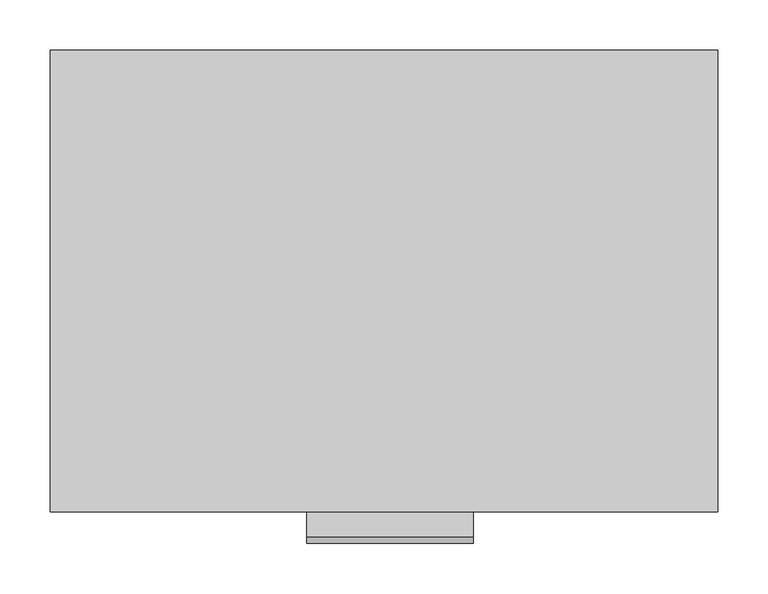
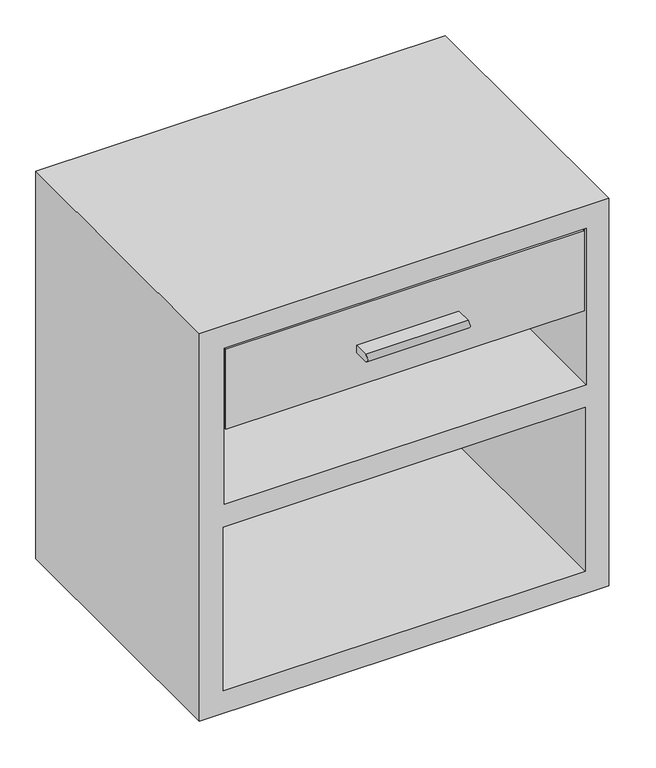
"""IFC4 building model written with IfcOpenShell, lengths in millimetres: furniture geometry, Livia_1_Drawer_Nightstand_20913 : Livia_1_Drawer_Nightstand_20913."""

from ifc_helpers import new_model, si_unit, frame, origin, place, context, project, spatial, faceted_brep, source, transform, mapped, element, save
from ifc_brep_helpers import plane_surface, extruded_surface, spline_curve, advanced_brep


def furniture_23f017af(model_context):
    return source(origin(), model_context, "Body", "SolidModel", [
        advanced_brep(
        [(-76.575761, -228.6, 552.45), (-76.575761, -228.6, 539.75), (-76.575761, -254.0, 539.75), (-76.575761, -254.0, 552.45), (88.524239, -228.6, 552.45), (88.524239, -254.0, 552.45), (88.524239, -254.0, 539.75), (88.524239, -228.6, 539.75)],
        [
            (0, 1),
            (1, 2),
            (2, 3, spline_curve(3, [(-76.575761, -254.0, 539.75), (-76.575761, -261.758833332, 543.737102154), (-76.575761, -261.758833332, 547.970435488), (-76.575761, -254.0, 552.45)], [4, 4], [0.0, 0.04350998662349671])),
            (3, 0),
            (4, 5),
            (5, 6, spline_curve(3, [(88.524239, -254.0, 552.45), (88.524239, -261.758833332, 547.970435488), (88.524239, -261.758833332, 543.737102154), (88.524239, -254.0, 539.75)], [4, 4], [0.0, 0.04350998662349671])),
            (6, 7),
            (7, 4),
            (0, 4),
            (7, 1),
            (6, 2),
            (5, 3),
        ],
        [
            plane_surface(frame((-76.575761, -228.6, 545.7306532), z_axis=(-1.0, 0.0, 0.0), x_axis=(0.0, -1.0, 0.0))),
            plane_surface(frame((88.524239, -228.6, 545.7306532), z_axis=(1.0, 0.0, 0.0), x_axis=(0.0, -1.0, 0.0))),
            plane_surface(frame((-76.575761, -228.6, 552.45), z_axis=(0.0, 1.0, 0.0), x_axis=(1.0, 0.0, 0.0))),
            plane_surface(frame((-76.575761, -228.6, 539.75), z_axis=(0.0, 0.0, -1.0), x_axis=(1.0, 0.0, 0.0))),
            extruded_surface(spline_curve(3, [(88.524239, -254.0, 539.75), (88.524239, -261.758833332, 543.737102154), (88.524239, -261.758833332, 547.970435488), (88.524239, -254.0, 552.45)], [4, 4], [0.0, 0.04350998662349671]), (-165.1, 0.0, 0.0), 165.1),
            plane_surface(frame((-76.575761, -254.0, 552.45), z_axis=(0.0, 0.0, 1.0), x_axis=(1.0, 0.0, 0.0))),
        ],
        [
            (0, [[1, 2, 3, 4]]),
            (1, [[5, 6, 7, 8]]),
            (2, [[-1, 9, -8, 10]]),
            (3, [[-2, -10, -7, 11]]),
            (4, [[-3, -11, -6, 12]]),
            (5, [[-4, -12, -5, -9]]),
        ],
    ),
        faceted_brep([(330.2, -228.6, 0.0), (330.2, -228.6, 660.4), (-330.2, -228.6, 660.4), (-330.2, -228.6, 0.0), (292.1, -228.6, 317.5), (292.1, -228.6, 38.1), (-292.1, -228.6, 38.1), (-292.1, -228.6, 317.5), (293.7115278, -228.6, 622.3), (293.7115278, -228.6, 355.6), (-290.4884722, -228.6, 355.6), (-290.4884722, -228.6, 622.3), (-287.3134722, -228.6, 482.6), (290.5365278, -228.6, 482.6), (290.5365278, -228.6, 619.125), (-287.3134722, -228.6, 619.125), (330.2, 228.6, 0.0), (-330.2, 228.6, 0.0), (-330.2, 228.6, 660.4), (330.2, 228.6, 660.4), (292.1, 228.6, 38.1), (292.1, 228.6, 317.5), (-292.1, 228.6, 317.5), (-292.1, 228.6, 38.1), (293.7115278, 228.6, 355.6), (293.7115278, 228.6, 482.6), (-290.4884722, 228.6, 482.6), (-290.4884722, 228.6, 355.6), (293.7115278, -223.8644244, 622.3), (293.7115278, -223.8644244, 482.6), (290.5365278, -223.8644244, 482.6), (-287.3134722, -223.8644244, 482.6), (-290.4884722, -223.8644244, 482.6), (-290.4884722, -223.8644244, 622.3), (-287.3134722, -223.8644244, 619.125), (290.5365278, -223.8644244, 619.125)], [[[0, 1, 2, 3], [4, 5, 6, 7], [8, 9, 10, 11]], [[12, 13, 14, 15]], [[16, 17, 18, 19], [20, 21, 22, 23], [24, 25, 26, 27]], [[1, 0, 16, 19]], [[2, 1, 19, 18]], [[3, 2, 18, 17]], [[0, 3, 17, 16]], [[20, 5, 4, 21]], [[21, 4, 7, 22]], [[22, 7, 6, 23]], [[5, 20, 23, 6]], [[24, 9, 8, 28, 29, 25]], [[26, 25, 29, 30, 13, 12, 31, 32]], [[10, 27, 26, 32, 33, 11]], [[9, 24, 27, 10]], [[33, 32, 31, 34, 35, 30, 29, 28]], [[34, 31, 12, 15]], [[35, 34, 15, 14]], [[30, 35, 14, 13]], [[33, 28, 8, 11]]]),
    ])


if __name__ == "__main__":
    model = new_model("IFC4")
    model_context = context("Model", 3, world=origin())
    ifc_project = project(units=[si_unit("LENGTHUNIT", "METRE", prefix="MILLI")], contexts=[model_context])
    site = spatial("IfcSite", under=ifc_project)
    building = spatial("IfcBuilding", under=site)
    placement = place(None, origin())
    furniture_shape = furniture_23f017af(model_context)
    element("IfcFurniture", 1, ObjectType="Livia_1_Drawer_Nightstand_20913 : Livia_1_Drawer_Nightstand_20913", at=placement, inside=building, context=model_context, shape_type="MappedRepresentation", body=[
        mapped(furniture_shape, transform((0.0, 0.0, 0.0), x_axis=(1.0, 0.0, 0.0), y_axis=(0.0, 1.0, 0.0), z_axis=(0.0, 0.0, 1.0))),
    ])
    save(model, "model.ifc")

# Revit data of these elements
# Type "Livia_1_Drawer_Nightstand_20913 : Livia_1_Drawer_Nightstand_20913"
#   Width = 0.6604 m
#   Depth = 0.4572 m
#   Side Table Material = none
#   Drawer Pull = none
#   Default Elevation = 0
